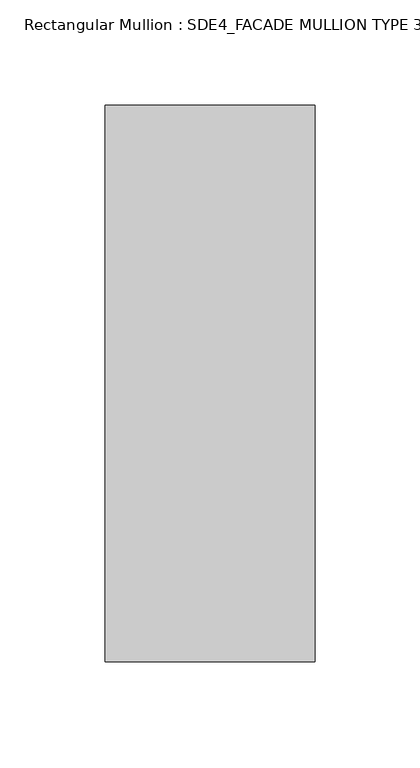
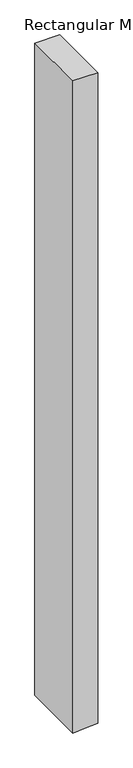
"""IFC4 building model written with IfcOpenShell, lengths in millimetres: member geometry, Rectangular Mullion : SDE4_FACADE MULLION TYPE 3."""

from ifc_helpers import new_model, si_unit, frame, origin, place, context, project, spatial, polyline, outline, extrude, source, transform, mapped, element, save


def rectangular_mullion_sde4_facade_mullion_type_3_5210846b(model_context):
    return source(origin(), model_context, "Body", "SweptSolid", [
        extrude(outline(polyline([(0.0, 50.0), (0.0, -50.0), (-2770.2451621, -50.0), (-2766.6475648, -3.056508), (-2762.5814857, 50.0), (0.0, 50.0)])), frame((0.0, -132.5, 0.0), z_axis=(0.0, 1.0, 0.0), x_axis=(0.0, 0.0, 1.0)), (0.0, 0.0, 1.0), 265.0),
    ])


if __name__ == "__main__":
    model = new_model("IFC4")
    model_context = context("Model", 3, world=origin())
    ifc_project = project(units=[si_unit("LENGTHUNIT", "METRE", prefix="MILLI")], contexts=[model_context])
    site = spatial("IfcSite", under=ifc_project)
    building = spatial("IfcBuilding", under=site)
    placement = place(None, origin())
    rectangular_mullion_sde4_facade_mullion_type_3_shape = rectangular_mullion_sde4_facade_mullion_type_3_5210846b(model_context)
    element("IfcMember", 1, ObjectType="Rectangular Mullion : SDE4_FACADE MULLION TYPE 3", at=placement, inside=building, context=model_context, shape_type="MappedRepresentation", body=[
        mapped(rectangular_mullion_sde4_facade_mullion_type_3_shape, transform((0.0, 0.0, 0.0), x_axis=(1.0, 0.0, 0.0), y_axis=(0.0, 1.0, 0.0), z_axis=(0.0, 0.0, 1.0))),
    ])
    save(model, "model.ifc")

# Revit data of these elements
# Type "Rectangular Mullion : SDE4_FACADE MULLION TYPE 3"
#   built-in parameter 1007322 = 0.869423 (stored number, unit not read)
#   built-in parameter 1007321 = 0.164042 (stored number, unit not read)
#   built-in parameter 1007320 = 0.164042 (stored number, unit not read)
